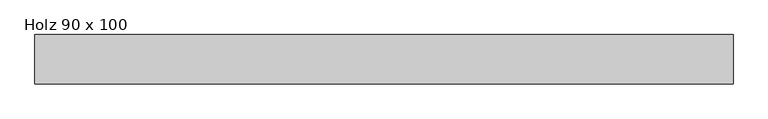
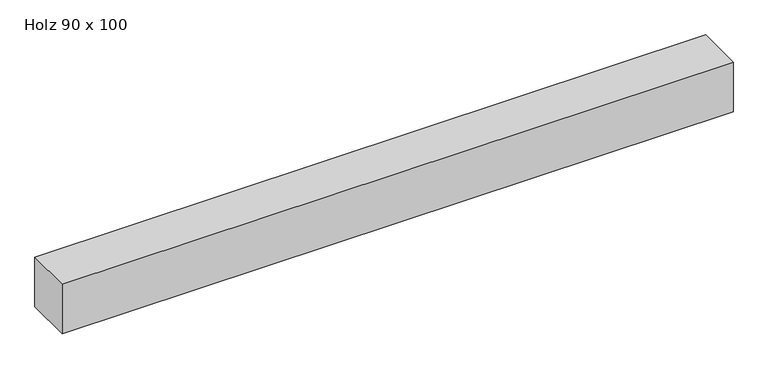
"""IFC4 building model written with IfcOpenShell, lengths in millimetres: beam geometry, Holz Träger - rechteckig : Holz 90 x 100."""

from ifc_helpers import new_model, si_unit, frame, origin, place, context, project, spatial, polyline, outline, extrude, source, transform, mapped, element, save


def holz_90_x_100_50d95c69(model_context):
    return source(origin(), model_context, "Body", "SweptSolid", [
        extrude(outline(polyline([(-638.5, -45.0), (-638.5, 45.0), (638.5, 45.0), (638.5, -45.0), (-638.5, -45.0)])), frame((0.0, 0.0, -50.0), z_axis=(0.0, 0.0, 1.0), x_axis=(1.0, 0.0, 0.0)), (0.0, 0.0, 1.0), 100.0),
    ])


if __name__ == "__main__":
    model = new_model("IFC4")
    model_context = context("Model", 3, world=origin())
    ifc_project = project(units=[si_unit("LENGTHUNIT", "METRE", prefix="MILLI")], contexts=[model_context])
    site = spatial("IfcSite", under=ifc_project)
    building = spatial("IfcBuilding", under=site)
    placement = place(None, origin())
    holz_90_x_100_shape = holz_90_x_100_50d95c69(model_context)
    element("IfcBeam", 1, ObjectType="Holz Träger - rechteckig : Holz 90 x 100", at=placement, inside=building, context=model_context, shape_type="MappedRepresentation", body=[
        mapped(holz_90_x_100_shape, transform((0.0, 0.0, 0.0), x_axis=(1.0, 0.0, 0.0), y_axis=(0.0, 1.0, 0.0), z_axis=(0.0, 0.0, 1.0))),
    ])
    save(model, "model.ifc")

# Revit data of these elements
# Type "Holz Träger - rechteckig : Holz 90 x 100"
#   Type Comments = "B/H=9/10cm"
#   Perimeter = 0.38 m²/m
#   Moment of Inertia strong axis = 750.00 cm⁴
#   Moment of Inertia weak axis = 607.50 cm⁴
#   Section Area = 90.0 cm²
#   Length [instance default] = 1.524 m
#   Height = 10.0 cm
#   Width = 9.0 cm
#   B = 0.090 m
#   H = 0.100 m
#   Structural Material = Holz - C 24 Cl.1
# Element 1 (IfcBeam, "Holz Träger - rechteckig : Holz 90 x 100")
#   Materials on its faces: "Holz - C 24 Cl.1"
# Materials
#   "Holz - C 24 Cl.1": class "Holz", colour RGB 218 191 173, transparency 0, Description = "Holz - C 24 Cl.1", Cost = 0
